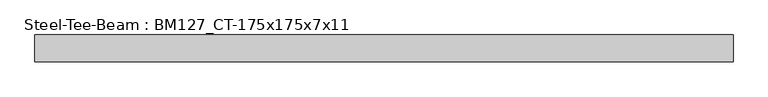
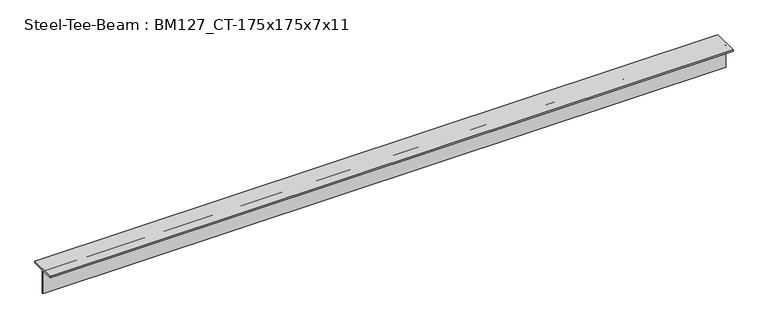
"""IFC4 building model written with IfcOpenShell, lengths in millimetres: beam geometry, Steel-Tee-Beam : BM127_CT-175x175x7x11."""

from ifc_helpers import new_model, si_unit, point, frame, frame_2d, origin, place, context, project, spatial, polyline, circle_curve, trimmed, segment, composite_curve, outline, extrude, source, transform, mapped, element, save


def steel_tee_beam_bm127_ct_175x175x7x11_df70e9a8(model_context):
    return source(origin(), model_context, "Body", "SweptSolid", [
        extrude(outline(composite_curve([segment(polyline([(87.5, 87.5), (87.5, 76.5), (17.5, 76.5)]), True, "CONTINUOUS"), segment(trimmed(circle_curve(frame_2d((17.5, 62.5)), 14.0), [point((17.5, 76.5))], [point((3.5, 62.5))], True, "CARTESIAN"), True, "CONTINUOUS"), segment(polyline([(3.5, 62.5), (3.5, -87.5), (-3.5, -87.5), (-3.5, 62.5)]), True, "CONTINUOUS"), segment(trimmed(circle_curve(frame_2d((-17.5, 62.5)), 14.0), [point((-3.5, 62.5))], [point((-17.5, 76.5))], True, "CARTESIAN"), True, "CONTINUOUS"), segment(polyline([(-17.5, 76.5), (-87.5, 76.5), (-87.5, 87.5), (87.5, 87.5)]), True, "CONTINUOUS")], self_intersect=False)), frame((-2375.7579713, 0.0, 0.0), z_axis=(1.0, 0.0, 0.0), x_axis=(0.0, 1.0, 0.0)), (0.0, 0.0, 1.0), 4573.2110535),
    ])


if __name__ == "__main__":
    model = new_model("IFC4")
    model_context = context("Model", 3, world=origin())
    ifc_project = project(units=[si_unit("LENGTHUNIT", "METRE", prefix="MILLI")], contexts=[model_context])
    site = spatial("IfcSite", under=ifc_project)
    building = spatial("IfcBuilding", under=site)
    placement = place(None, origin())
    steel_tee_beam_bm127_ct_175x175x7x11_shape = steel_tee_beam_bm127_ct_175x175x7x11_df70e9a8(model_context)
    element("IfcBeam", 1, ObjectType="Steel-Tee-Beam : BM127_CT-175x175x7x11", at=placement, inside=building, context=model_context, shape_type="MappedRepresentation", body=[
        mapped(steel_tee_beam_bm127_ct_175x175x7x11_shape, transform((0.0, 0.0, 0.0), x_axis=(1.0, 0.0, 0.0), y_axis=(0.0, 1.0, 0.0), z_axis=(0.0, 0.0, 1.0))),
    ])
    save(model, "model.ifc")

# Revit data of these elements
# Type "Steel-Tee-Beam : BM127_CT-175x175x7x11"
#   Section Area = 31.57 cm²
#   Mass per Unit Length = 24.80 kg/m
#   Length [instance default] = 1524 mm
#   bf = 175 mm
#   d = 175 mm
#   k = 25 mm
#   kr = 14 mm
#   tf = 11 mm
#   tw = 7 mm
#   hec_material4 [instance default] = none
#   hec_material3 [instance default] = none
#   hec_material2 [instance default] = none
#   hec_material1 [instance default] = none
#   Structural Material [instance default] = Steel, 45-345
#   Assembly Code = ""
# Element 1 (IfcBeam, "Steel-Tee-Beam : BM127_CT-175x175x7x11")
#   hec_material3 = F01AC000-00002_Building/Shelter Fire Proofing Work_Intumescent Coating Type_1 hr. rating (UL 1709))
#   hec_material1 = S03AA029-00001_Main Steel Structure Erection Work_Shelter/Building_Light Steel
#   Structural Material = S01AA003-00001_Main Steel Structure Fabrication Work_Shelter/Building_Light Steel - Standard
#   Materials on its faces: "S01AA003-00001_Main Steel Structure Fabrication Work_Shelter/Building_Light Steel - Standard"
# Materials
#   "Steel, 45-345": class "Metal", colour RGB 189 187 185, transparency 0, Description = "Steel 345 MPa", Cost = 0
#   "S01AA003-00001_Main Steel Structure Fabrication Work_Shelter/Building_Light Steel - Standard": class "Metal", colour RGB 120 120 120, transparency 0, Comments = "(30KG/M>Weight)", Description = "Structural steel 50ksi", W00) Work Master Code = "S01AA003-00001", W01) Work Master_Lv1 = "Main Steel Structure Fabrication Work", W02) Work Master_Lv2 = "Shelter/Building", W03) Work Master_Spec.1 = "Light Steel - Standard (30KG/M>Weight)", Cost = 0
#   "F01AC000-00002_Building/Shelter Fire Proofing Work_Intumescent Coating Type_1 hr. rating (UL 1709))": class "Metal", colour RGB 255 128 128, transparency 0, Description = "Paint finished steel", W00) Work Master Code = "F01AC000-00002", W01) Work Master_Lv1 = "Building/Shelter Fire Proofing Work", W02) Work Master_Lv2 = "Intumescent Coating Type", W03) Work Master_Spec.1 = "1 hr. rating (UL 1709)", Cost = 0
#   "S03AA029-00001_Main Steel Structure Erection Work_Shelter/Building_Light Steel": class "Metal", colour RGB 120 120 120, transparency 0, Comments = "(30KG/M>Weight)", Description = "Structural steel 50ksi", W00) Work Master Code = "S03AA029-00001", W01) Work Master_Lv1 = "Main Steel Structure Erection Work", W02) Work Master_Lv2 = "Shelter/Building", W03) Work Master_Spec.1 = "Light Steel (30KG/M>Weight)", Cost = 0
